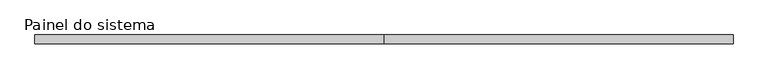
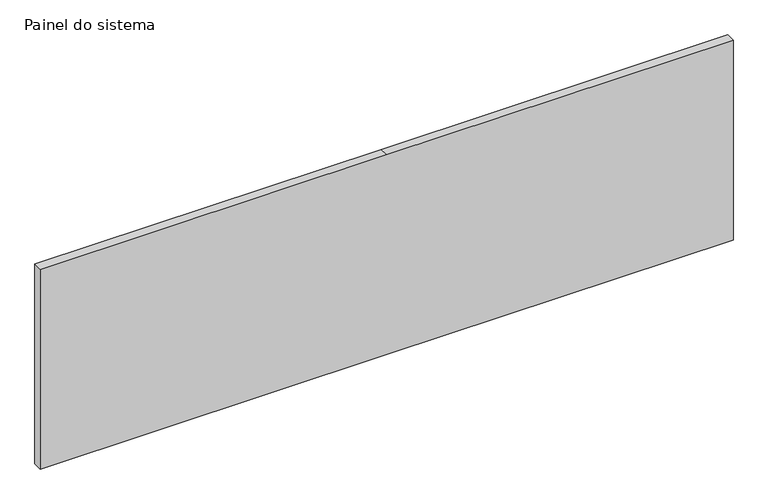
"""IFC4 building model written with IfcOpenShell, lengths in millimetres: plate geometry, Painel do sistema : Envidraçado."""

import ifcopenshell
import ifcopenshell.guid

model = None  # the IFC model being written
_history = None  # IfcOwnerHistory: only IFC2X3 demands one
_inside = {}  # id of a spatial element -> (the spatial element, [elements in it])
_under = {}  # id of a project, library or spatial element -> (it, [spatial elements below it])
_declared = {}  # id of a project -> (the project, [libraries it declares])
_typed = {}  # id of a type object -> (the type object, [elements of that type])
_made_of = {}  # id of a material, layer set ... -> (it, [elements and type objects made of it])


def new_model(schema):
    """Start an empty IFC model of exactly this schema.

    Asked for "IFC4X3", IfcOpenShell would pick the latest addendum, in which some entities
    have other attributes; the version numbers below select the first issue.
    IFC2X3 requires an IfcOwnerHistory on every rooted entity: one is made here for all.
    """
    global model, _history
    if schema == "IFC4X3":
        model = ifcopenshell.file(schema_version=(4, 3, 0, 0))
    else:
        model = ifcopenshell.file(schema=schema)
    _inside.clear()
    _under.clear()
    _declared.clear()
    _typed.clear()
    _made_of.clear()
    _history = None
    if model.schema == "IFC2X3":
        org = make("IfcOrganization", Name="unknown")
        user = make(
            "IfcPersonAndOrganization",
            ThePerson=make("IfcPerson", FamilyName="unknown"),
            TheOrganization=org,
        )
        app = make(
            "IfcApplication",
            ApplicationDeveloper=org,
            Version="unknown",
            ApplicationFullName="unknown",
            ApplicationIdentifier="unknown",
        )
        _history = make(
            "IfcOwnerHistory",
            OwningUser=user,
            OwningApplication=app,
            ChangeAction="ADDED",
            CreationDate=0,
        )
    return model


def make(cls, **values):
    """One entity of the class cls with the attributes given. An attribute that is None is left unset."""
    return model.create_entity(
        cls, **{name: value for name, value in values.items() if value is not None}
    )


def rooted(cls, **values):
    """An entity with a GlobalId (a new one), such as an element, a storey or a relation."""
    return make(cls, GlobalId=ifcopenshell.guid.new(), OwnerHistory=_history, **values)


def si_unit(unit_type, name, prefix=None):
    """IfcSIUnit, for example si_unit("LENGTHUNIT", "METRE", prefix="MILLI")."""
    return make("IfcSIUnit", UnitType=unit_type, Prefix=prefix, Name=name)


def assignment(units):
    """IfcUnitAssignment: the units of a project."""
    return None if units is None else make("IfcUnitAssignment", Units=units)


def point(xyz):
    """IfcCartesianPoint."""
    return None if xyz is None else make("IfcCartesianPoint", Coordinates=xyz)


def direction(xyz):
    """IfcDirection."""
    return None if xyz is None else make("IfcDirection", DirectionRatios=xyz)


def frame(location, z_axis=None, x_axis=None):
    """IfcAxis2Placement3D, a coordinate frame: its origin and axes. An axis left out is left unset."""
    return make(
        "IfcAxis2Placement3D",
        Location=point(location),
        Axis=direction(z_axis),
        RefDirection=direction(x_axis),
    )


def origin():
    """The frame at (0, 0, 0) with its axes left unset."""
    return frame((0.0, 0.0, 0.0))


def place(relative_to, where):
    """IfcLocalPlacement: puts the frame where relative to a parent placement (None: the world)."""
    return make(
        "IfcLocalPlacement", PlacementRelTo=relative_to, RelativePlacement=where
    )


def context(
    kind, dimensions, precision=None, world=None, true_north=None, identifier=None
):
    """IfcGeometricRepresentationContext, for example the 3D "Model" context."""
    return make(
        "IfcGeometricRepresentationContext",
        ContextIdentifier=identifier,
        ContextType=kind,
        CoordinateSpaceDimension=dimensions,
        Precision=precision,
        WorldCoordinateSystem=world,
        TrueNorth=true_north,
    )


def project(units=None, contexts=None):
    """IfcProject with its units and contexts."""
    return rooted(
        "IfcProject",
        Name="project",
        RepresentationContexts=contexts,
        UnitsInContext=assignment(units),
    )


def spatial(cls, under=None, at=None, **own):
    """A site, building, storey or space (cls), placed at a placement, below another one or the project."""
    s = rooted(cls, ObjectPlacement=at, **own)
    if under is not None:
        _under.setdefault(under.id(), (under, []))[1].append(s)
    return s


def polyline(points):
    """IfcPolyline through the points."""
    return make("IfcPolyline", Points=[point(p) for p in points])


def outline(outer, holes=None, kind="AREA"):
    """IfcArbitraryClosedProfileDef: a profile drawn as a closed curve; with holes, ...WithVoids."""
    if holes is None:
        return make("IfcArbitraryClosedProfileDef", ProfileType=kind, OuterCurve=outer)
    return make(
        "IfcArbitraryProfileDefWithVoids",
        ProfileType=kind,
        OuterCurve=outer,
        InnerCurves=holes,
    )


def extrude(swept, where, along, depth):
    """IfcExtrudedAreaSolid: the profile swept, set in the frame where, extruded along a direction by depth."""
    return make(
        "IfcExtrudedAreaSolid",
        SweptArea=swept,
        Position=where,
        ExtrudedDirection=direction(along),
        Depth=depth,
    )


def shape(context_of_items, identifier, shape_type, items):
    """IfcShapeRepresentation: the items that make up one representation, for example the "Body"."""
    return make(
        "IfcShapeRepresentation",
        ContextOfItems=context_of_items,
        RepresentationIdentifier=identifier,
        RepresentationType=shape_type,
        Items=items,
    )


def source(mapping_origin, context_of_items, identifier, shape_type, items):
    """IfcRepresentationMap: a shape defined once, which mapped items show again and again."""
    return make(
        "IfcRepresentationMap",
        MappingOrigin=mapping_origin,
        MappedRepresentation=shape(context_of_items, identifier, shape_type, items),
    )


def transform(
    local_origin,
    x_axis=None,
    y_axis=None,
    z_axis=None,
    scale=None,
    scale2=None,
    scale3=None,
    uniform=True,
):
    """IfcCartesianTransformationOperator3D, or its non-uniform kind. x_axis, y_axis, z_axis: its Axis1, 2, 3."""
    if uniform:
        return make(
            "IfcCartesianTransformationOperator3D",
            Axis1=direction(x_axis),
            Axis2=direction(y_axis),
            LocalOrigin=point(local_origin),
            Scale=scale,
            Axis3=direction(z_axis),
        )
    return make(
        "IfcCartesianTransformationOperator3DnonUniform",
        Axis1=direction(x_axis),
        Axis2=direction(y_axis),
        LocalOrigin=point(local_origin),
        Scale=scale,
        Axis3=direction(z_axis),
        Scale2=scale2,
        Scale3=scale3,
    )


def mapped(mapping_source, mapping_target):
    """IfcMappedItem: shows the shape of a source again, moved by a transform."""
    return make(
        "IfcMappedItem", MappingSource=mapping_source, MappingTarget=mapping_target
    )


def made_of(thing, what):
    """Note that an element or type object is made of a material, layer set ...; save() writes the relation."""
    if what is not None:
        _made_of.setdefault(what.id(), (what, []))[1].append(thing)
    return thing


def element(
    cls,
    number,
    at=None,
    inside=None,
    cuts=None,
    type_object=None,
    material=None,
    context=None,
    identifier="Body",
    shape_type=None,
    held_by="IfcProductDefinitionShape",
    body=None,
    shapes=None,
    **own,
):
    """One element of the class cls, such as IfcWall. Its Tag is "e" and its number.

    at: its placement. inside: the storey or other place that contains it. cuts: it is an
    opening in that element (IfcRelVoidsElement). A single representation is given by context,
    identifier, shape_type and body (its items); several are given by shapes. held_by: the class
    of the entity that holds the representations. save() writes the other relations.
    """
    e = rooted(cls, Tag="e%d" % number, ObjectPlacement=at, **own)
    if body is not None:
        shapes = [shape(context, identifier, shape_type, body)]
    if shapes is not None:
        e.Representation = make(held_by, Representations=shapes)
    if inside is not None:
        _inside.setdefault(inside.id(), (inside, []))[1].append(e)
    if cuts is not None:
        rooted(
            "IfcRelVoidsElement", RelatingBuildingElement=cuts, RelatedOpeningElement=e
        )
    if type_object is not None:
        _typed.setdefault(type_object.id(), (type_object, []))[1].append(e)
    return made_of(e, material)


def aggregate(whole, parts):
    """IfcRelAggregates: a whole, such as a stair, and the parts it consists of."""
    return rooted("IfcRelAggregates", RelatingObject=whole, RelatedObjects=parts)


def save(model, path):
    """Write the relations noted so far, then the file.

    IfcRelAggregates (storeys below a building ...), IfcRelContainedInSpatialStructure (elements
    in a storey), IfcRelDefinesByType, IfcRelAssociatesMaterial and IfcRelDeclares: one each for
    every whole, place, type object, material and project.
    """
    for whole, parts in _under.values():
        aggregate(whole, parts)
    for where, things in _inside.values():
        rooted(
            "IfcRelContainedInSpatialStructure",
            RelatedElements=things,
            RelatingStructure=where,
        )
    for kind, things in _typed.values():
        rooted("IfcRelDefinesByType", RelatedObjects=things, RelatingType=kind)
    for what, things in _made_of.values():
        rooted("IfcRelAssociatesMaterial", RelatedObjects=things, RelatingMaterial=what)
    for by, libraries in _declared.values():
        rooted("IfcRelDeclares", RelatingContext=by, RelatedDefinitions=libraries)
    model.write(path)


def painel_do_sistema_f930648b(model_context):
    return source(origin(), model_context, "Body", "SweptSolid", [
        extrude(outline(polyline([(0.0, -966.7099999), (0.0, 0.0), (0.0, 966.7099999), (590.0, 966.7099999), (590.0, 0.0), (590.0, -966.7099999), (0.0, -966.7099999)])), frame((0.0, -49.5, 0.0), z_axis=(0.0, 1.0, 0.0), x_axis=(0.0, 0.0, 1.0)), (0.0, 0.0, 1.0), 25.0),
    ])


if __name__ == "__main__":
    model = new_model("IFC4")
    model_context = context("Model", 3, world=origin())
    ifc_project = project(units=[si_unit("LENGTHUNIT", "METRE", prefix="MILLI")], contexts=[model_context])
    site = spatial("IfcSite", under=ifc_project)
    building = spatial("IfcBuilding", under=site)
    placement = place(None, origin())
    painel_do_sistema_shape = painel_do_sistema_f930648b(model_context)
    element("IfcPlate", 1, ObjectType="Painel do sistema : Envidraçado", at=placement, inside=building, context=model_context, shape_type="MappedRepresentation", body=[
        mapped(painel_do_sistema_shape, transform((0.0, 0.0, 0.0), x_axis=(1.0, 0.0, 0.0), y_axis=(0.0, 1.0, 0.0), z_axis=(0.0, 0.0, 1.0))),
    ])
    save(model, "model.ifc")

# Revit data of these elements
# Type "Painel do sistema : Envidraçado"
#   Construction Type Id = "GSP4R"
#   Analytic Construction = "Vidraça única Pilkington 1/8 pol"
#   Visual Light Transmittance = 0.9
#   Solar Heat Gain Coefficient = 0.86
#   Heat Transfer Coefficient (U) = 6.7069 W/(m²·K)
# Element 1 (IfcPlate, "Painel do sistema : Envidraçado")
#   Materials on its faces: ".VIDRO GENÉRICO"
# Materials
#   ".VIDRO GENÉRICO": class ".CC_VIDRO", colour RGB 0 128 192, transparency 0.9, Description = "Vidro comum", Cost = 0
